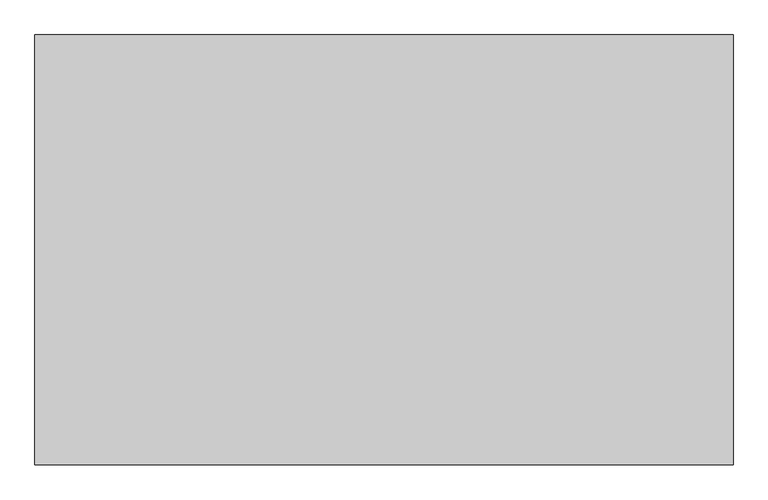
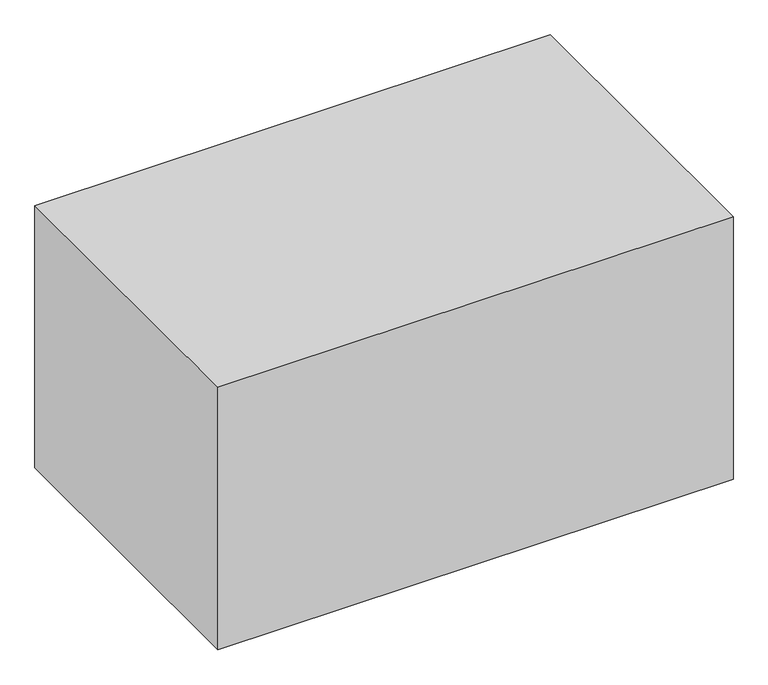
"""IFC4 building model written with IfcOpenShell, lengths in millimetres: proxy geometry, Space Planning Box_hec : Space Planning Box_hec."""

import ifcopenshell
import ifcopenshell.guid

model = None  # the IFC model being written
_history = None  # IfcOwnerHistory: only IFC2X3 demands one
_inside = {}  # id of a spatial element -> (the spatial element, [elements in it])
_under = {}  # id of a project, library or spatial element -> (it, [spatial elements below it])
_declared = {}  # id of a project -> (the project, [libraries it declares])
_typed = {}  # id of a type object -> (the type object, [elements of that type])
_made_of = {}  # id of a material, layer set ... -> (it, [elements and type objects made of it])


def new_model(schema):
    """Start an empty IFC model of exactly this schema.

    Asked for "IFC4X3", IfcOpenShell would pick the latest addendum, in which some entities
    have other attributes; the version numbers below select the first issue.
    IFC2X3 requires an IfcOwnerHistory on every rooted entity: one is made here for all.
    """
    global model, _history
    if schema == "IFC4X3":
        model = ifcopenshell.file(schema_version=(4, 3, 0, 0))
    else:
        model = ifcopenshell.file(schema=schema)
    _inside.clear()
    _under.clear()
    _declared.clear()
    _typed.clear()
    _made_of.clear()
    _history = None
    if model.schema == "IFC2X3":
        org = make("IfcOrganization", Name="unknown")
        user = make(
            "IfcPersonAndOrganization",
            ThePerson=make("IfcPerson", FamilyName="unknown"),
            TheOrganization=org,
        )
        app = make(
            "IfcApplication",
            ApplicationDeveloper=org,
            Version="unknown",
            ApplicationFullName="unknown",
            ApplicationIdentifier="unknown",
        )
        _history = make(
            "IfcOwnerHistory",
            OwningUser=user,
            OwningApplication=app,
            ChangeAction="ADDED",
            CreationDate=0,
        )
    return model


def make(cls, **values):
    """One entity of the class cls with the attributes given. An attribute that is None is left unset."""
    return model.create_entity(
        cls, **{name: value for name, value in values.items() if value is not None}
    )


def rooted(cls, **values):
    """An entity with a GlobalId (a new one), such as an element, a storey or a relation."""
    return make(cls, GlobalId=ifcopenshell.guid.new(), OwnerHistory=_history, **values)


def si_unit(unit_type, name, prefix=None):
    """IfcSIUnit, for example si_unit("LENGTHUNIT", "METRE", prefix="MILLI")."""
    return make("IfcSIUnit", UnitType=unit_type, Prefix=prefix, Name=name)


def assignment(units):
    """IfcUnitAssignment: the units of a project."""
    return None if units is None else make("IfcUnitAssignment", Units=units)


def point(xyz):
    """IfcCartesianPoint."""
    return None if xyz is None else make("IfcCartesianPoint", Coordinates=xyz)


def direction(xyz):
    """IfcDirection."""
    return None if xyz is None else make("IfcDirection", DirectionRatios=xyz)


def frame(location, z_axis=None, x_axis=None):
    """IfcAxis2Placement3D, a coordinate frame: its origin and axes. An axis left out is left unset."""
    return make(
        "IfcAxis2Placement3D",
        Location=point(location),
        Axis=direction(z_axis),
        RefDirection=direction(x_axis),
    )


def origin():
    """The frame at (0, 0, 0) with its axes left unset."""
    return frame((0.0, 0.0, 0.0))


def origin_with_axes():
    """The frame at (0, 0, 0) with the z axis (0, 0, 1) and the x axis (1, 0, 0) written out."""
    return frame((0.0, 0.0, 0.0), z_axis=(0.0, 0.0, 1.0), x_axis=(1.0, 0.0, 0.0))


def place(relative_to, where):
    """IfcLocalPlacement: puts the frame where relative to a parent placement (None: the world)."""
    return make(
        "IfcLocalPlacement", PlacementRelTo=relative_to, RelativePlacement=where
    )


def context(
    kind, dimensions, precision=None, world=None, true_north=None, identifier=None
):
    """IfcGeometricRepresentationContext, for example the 3D "Model" context."""
    return make(
        "IfcGeometricRepresentationContext",
        ContextIdentifier=identifier,
        ContextType=kind,
        CoordinateSpaceDimension=dimensions,
        Precision=precision,
        WorldCoordinateSystem=world,
        TrueNorth=true_north,
    )


def project(units=None, contexts=None):
    """IfcProject with its units and contexts."""
    return rooted(
        "IfcProject",
        Name="project",
        RepresentationContexts=contexts,
        UnitsInContext=assignment(units),
    )


def spatial(cls, under=None, at=None, **own):
    """A site, building, storey or space (cls), placed at a placement, below another one or the project."""
    s = rooted(cls, ObjectPlacement=at, **own)
    if under is not None:
        _under.setdefault(under.id(), (under, []))[1].append(s)
    return s


def polyline(points):
    """IfcPolyline through the points."""
    return make("IfcPolyline", Points=[point(p) for p in points])


def outline(outer, holes=None, kind="AREA"):
    """IfcArbitraryClosedProfileDef: a profile drawn as a closed curve; with holes, ...WithVoids."""
    if holes is None:
        return make("IfcArbitraryClosedProfileDef", ProfileType=kind, OuterCurve=outer)
    return make(
        "IfcArbitraryProfileDefWithVoids",
        ProfileType=kind,
        OuterCurve=outer,
        InnerCurves=holes,
    )


def extrude(swept, where, along, depth):
    """IfcExtrudedAreaSolid: the profile swept, set in the frame where, extruded along a direction by depth."""
    return make(
        "IfcExtrudedAreaSolid",
        SweptArea=swept,
        Position=where,
        ExtrudedDirection=direction(along),
        Depth=depth,
    )


def shape(context_of_items, identifier, shape_type, items):
    """IfcShapeRepresentation: the items that make up one representation, for example the "Body"."""
    return make(
        "IfcShapeRepresentation",
        ContextOfItems=context_of_items,
        RepresentationIdentifier=identifier,
        RepresentationType=shape_type,
        Items=items,
    )


def source(mapping_origin, context_of_items, identifier, shape_type, items):
    """IfcRepresentationMap: a shape defined once, which mapped items show again and again."""
    return make(
        "IfcRepresentationMap",
        MappingOrigin=mapping_origin,
        MappedRepresentation=shape(context_of_items, identifier, shape_type, items),
    )


def transform(
    local_origin,
    x_axis=None,
    y_axis=None,
    z_axis=None,
    scale=None,
    scale2=None,
    scale3=None,
    uniform=True,
):
    """IfcCartesianTransformationOperator3D, or its non-uniform kind. x_axis, y_axis, z_axis: its Axis1, 2, 3."""
    if uniform:
        return make(
            "IfcCartesianTransformationOperator3D",
            Axis1=direction(x_axis),
            Axis2=direction(y_axis),
            LocalOrigin=point(local_origin),
            Scale=scale,
            Axis3=direction(z_axis),
        )
    return make(
        "IfcCartesianTransformationOperator3DnonUniform",
        Axis1=direction(x_axis),
        Axis2=direction(y_axis),
        LocalOrigin=point(local_origin),
        Scale=scale,
        Axis3=direction(z_axis),
        Scale2=scale2,
        Scale3=scale3,
    )


def mapped(mapping_source, mapping_target):
    """IfcMappedItem: shows the shape of a source again, moved by a transform."""
    return make(
        "IfcMappedItem", MappingSource=mapping_source, MappingTarget=mapping_target
    )


def made_of(thing, what):
    """Note that an element or type object is made of a material, layer set ...; save() writes the relation."""
    if what is not None:
        _made_of.setdefault(what.id(), (what, []))[1].append(thing)
    return thing


def element(
    cls,
    number,
    at=None,
    inside=None,
    cuts=None,
    type_object=None,
    material=None,
    context=None,
    identifier="Body",
    shape_type=None,
    held_by="IfcProductDefinitionShape",
    body=None,
    shapes=None,
    **own,
):
    """One element of the class cls, such as IfcWall. Its Tag is "e" and its number.

    at: its placement. inside: the storey or other place that contains it. cuts: it is an
    opening in that element (IfcRelVoidsElement). A single representation is given by context,
    identifier, shape_type and body (its items); several are given by shapes. held_by: the class
    of the entity that holds the representations. save() writes the other relations.
    """
    e = rooted(cls, Tag="e%d" % number, ObjectPlacement=at, **own)
    if body is not None:
        shapes = [shape(context, identifier, shape_type, body)]
    if shapes is not None:
        e.Representation = make(held_by, Representations=shapes)
    if inside is not None:
        _inside.setdefault(inside.id(), (inside, []))[1].append(e)
    if cuts is not None:
        rooted(
            "IfcRelVoidsElement", RelatingBuildingElement=cuts, RelatedOpeningElement=e
        )
    if type_object is not None:
        _typed.setdefault(type_object.id(), (type_object, []))[1].append(e)
    return made_of(e, material)


def aggregate(whole, parts):
    """IfcRelAggregates: a whole, such as a stair, and the parts it consists of."""
    return rooted("IfcRelAggregates", RelatingObject=whole, RelatedObjects=parts)


def save(model, path):
    """Write the relations noted so far, then the file.

    IfcRelAggregates (storeys below a building ...), IfcRelContainedInSpatialStructure (elements
    in a storey), IfcRelDefinesByType, IfcRelAssociatesMaterial and IfcRelDeclares: one each for
    every whole, place, type object, material and project.
    """
    for whole, parts in _under.values():
        aggregate(whole, parts)
    for where, things in _inside.values():
        rooted(
            "IfcRelContainedInSpatialStructure",
            RelatedElements=things,
            RelatingStructure=where,
        )
    for kind, things in _typed.values():
        rooted("IfcRelDefinesByType", RelatedObjects=things, RelatingType=kind)
    for what, things in _made_of.values():
        rooted("IfcRelAssociatesMaterial", RelatedObjects=things, RelatingMaterial=what)
    for by, libraries in _declared.values():
        rooted("IfcRelDeclares", RelatingContext=by, RelatedDefinitions=libraries)
    model.write(path)


def generic_models_8c4134a9(model_context):
    return source(origin(), model_context, "Body", "SweptSolid", [
        extrude(outline(polyline([(3250.0, 2000.0), (3250.0, -2000.0), (-3250.0, -2000.0), (-3250.0, 2000.0), (3250.0, 2000.0)])), origin_with_axes(), (0.0, 0.0, 1.0), 3500.0),
    ])


if __name__ == "__main__":
    model = new_model("IFC4")
    model_context = context("Model", 3, world=origin())
    ifc_project = project(units=[si_unit("LENGTHUNIT", "METRE", prefix="MILLI")], contexts=[model_context])
    site = spatial("IfcSite", under=ifc_project)
    building = spatial("IfcBuilding", under=site)
    placement = place(None, origin())
    generic_models_shape = generic_models_8c4134a9(model_context)
    element("IfcBuildingElementProxy", 1, Name="Space Planning Box_hec : Space Planning Box_hec", ObjectType="Space Planning Box_hec : Space Planning Box_hec", at=placement, inside=building, context=model_context, shape_type="MappedRepresentation", body=[
        mapped(generic_models_shape, transform((0.0, 0.0, 0.0), x_axis=(1.0, 0.0, 0.0), y_axis=(0.0, 1.0, 0.0), z_axis=(0.0, 0.0, 1.0))),
    ])
    save(model, "model.ifc")

# Revit data of these elements
# Type "Space Planning Box_hec : Space Planning Box_hec"
#   Type Comments = "..."
#   Room Name [instance default] = "?"
#   Interior Finish [instance default] = ""
#   Exterior Finish [instance default] = ""
#   Department [instance default] = ""
#   Assembly Code = "..."
#   ceiling height [instance default] = 0
#   Width [instance default] = 1524 mm
#   Program Area [instance default] = 0.00 m²
#   Length [instance default] = 1524 mm
#   Height [instance default] = 1524 mm
#   Area [instance default] = 2.32258 m²
#   Fill Color [instance default] = Cyan
#   Default Elevation = 0
# Element 1 (IfcBuildingElementProxy, "Space Planning Box_hec : Space Planning Box_hec")
#   Room Name = "Manager Office-1"
#   Exterior Finish = "RF1..N/A,,EW1..N/A..N/A"
#   Department = "AR"
#   Width = 6500 mm
#   Program Area = 26.00 m²
#   Length = 4000 mm
#   Height = 3500 mm
#   Area = 26.00 m²
#   Materials on its faces: "Cyan"
# Materials
#   "Cyan": class "Generic", colour RGB 0 255 255, transparency 0.2, Cost = 0
